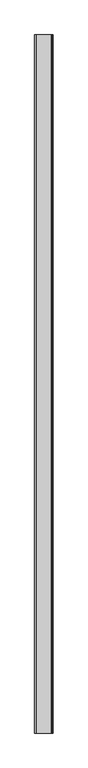
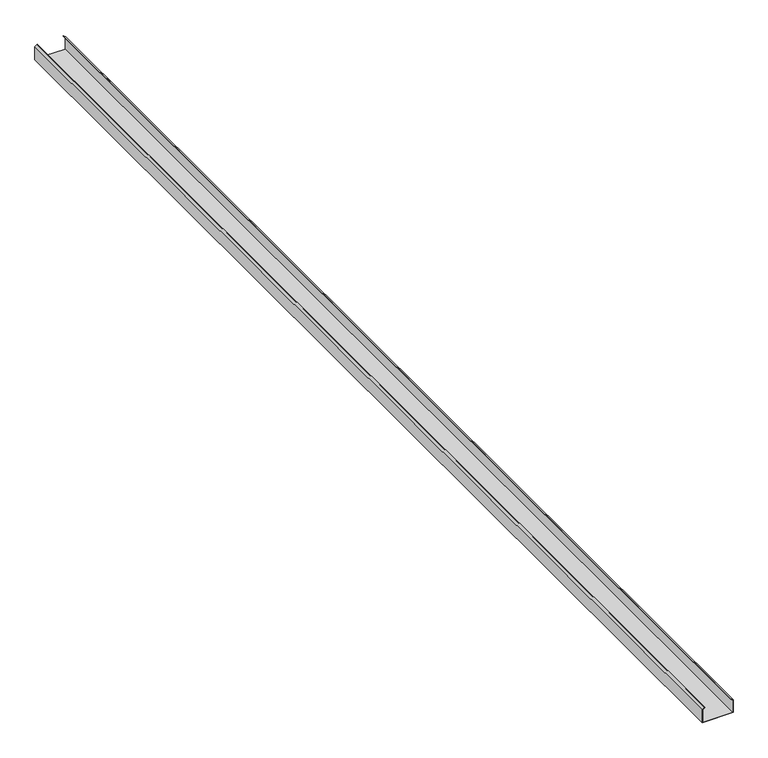
"""IFC4 building model written with IfcOpenShell, lengths in millimetres: proxy geometry, Generic Models 7:Generic Models 1:1:Generic Models 1:1 : Generic Models 7:Generic Models 1:337419:40 : Generic Models 7:Generic Models 1:1:Generic Models 1:1 : Generic Models 7:Generic Models 1:337419:306201."""

from ifc_helpers import new_model, si_unit, frame, origin, place, context, project, spatial, polyline, outline, extrude, source, transform, mapped, element, save


def generic_models_d9c83517(model_context):
    return source(origin(), model_context, "Body", "SweptSolid", [
        extrude(outline(polyline([(2446.5359375, 667293.3117239), (2446.5359375, 667496.5117239), (2535.4359375, 667496.5117239), (2547.6810414, 667481.9185773), (2545.5528742, 667480.132833), (2534.1404765, 667493.7335989), (2449.3140625, 667493.7335989), (2449.3140625, 667296.0898489), (2534.1404765, 667296.0898489), (2545.5528742, 667309.6906149), (2547.6810414, 667307.9048706), (2535.4359375, 667293.3117239), (2446.5359375, 667293.3117239)])), frame((0.0, -507687.0163841, 0.0), z_axis=(0.0, 1.0, 0.0), x_axis=(0.0, 0.0, 1.0)), (0.0, 0.0, 1.0), 7653.1810262),
    ])


if __name__ == "__main__":
    model = new_model("IFC4")
    model_context = context("Model", 3, world=origin())
    ifc_project = project(units=[si_unit("LENGTHUNIT", "METRE", prefix="MILLI")], contexts=[model_context])
    site = spatial("IfcSite", under=ifc_project)
    building = spatial("IfcBuilding", under=site)
    placement = place(None, origin())
    generic_models_shape = generic_models_d9c83517(model_context)
    element("IfcBuildingElementProxy", 1, Name="Generic Models 7:Generic Models 1:1:Generic Models 1:1 : Generic Models 7:Generic Models 1:337419:40 : Generic Models 7:Generic Models 1:1:Generic Models 1:1 : Generic Models 7:Generic Models 1:337419:306201", ObjectType="Generic Models 7:Generic Models 1:1:Generic Models 1:1 : Generic Models 7:Generic Models 1:337419:40 : Generic Models 7:Generic Models 1:1:Generic Models 1:1 : Generic Models 7:Generic Models 1:337419:306201", at=placement, inside=building, context=model_context, shape_type="MappedRepresentation", body=[
        mapped(generic_models_shape, transform((0.0, 0.0, 0.0), x_axis=(1.0, 0.0, 0.0), y_axis=(0.0, 1.0, 0.0), z_axis=(0.0, 0.0, 1.0))),
    ])
    save(model, "model.ifc")

# Revit data of these elements
# Type "Generic Models 7:Generic Models 1:1:Generic Models 1:1 : Generic Models 7:Generic Models 1:337419:40 : Generic Models 7:Generic Models 1:1:Generic Models 1:1 : Generic Models 7:Generic Models 1:337419:306201"
#   NameOverride = "Generic Models 7:Generic Models 1:1:Generic Models 1:1 : Generic Models 7:Generic Models 1:337419:306201"
#   ObjectTypeOverride = "Generic Models 1:1 : Generic Models 7:Generic Models 1:337419"
#   Reference = "Generic Models 1"
#   Tag = "306201"
# Element 1 (IfcBuildingElementProxy, "Generic Models 7:Generic Models 1:1:Generic Models 1:1 : Generic Models 7:Generic Models 1:337419:40 : Generic Models 7:Generic Models 1:1:Generic Models 1:1 : Generic Models 7:Generic Models 1:337419:306201")
#   Materials on its faces: "CEE' SECTION (8.0x3.5C - SEE STRUCT. DWGS)"
# Materials
#   "CEE' SECTION (8.0x3.5C - SEE STRUCT. DWGS)": class "Unassigned", colour RGB 210 209 208, transparency 0, Keynote = "M05121300.02", Cost = 0
